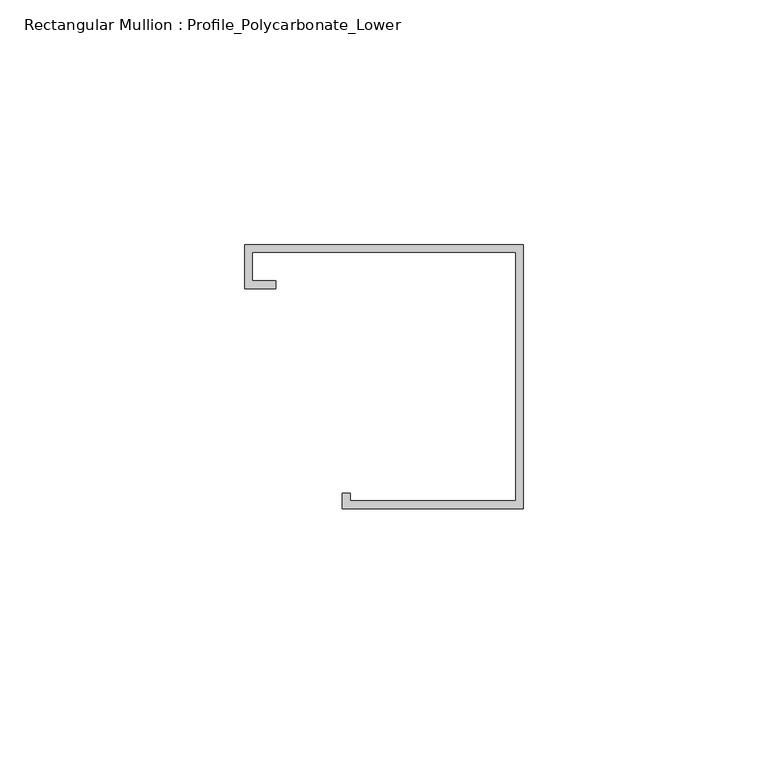
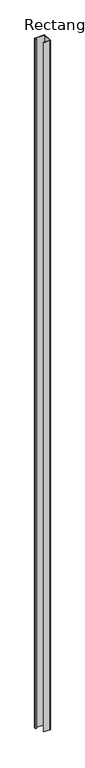
"""IFC4 building model written with IfcOpenShell, lengths in millimetres: member geometry, Rectangular Mullion : Profile_Polycarbonate_Lower."""

import ifcopenshell
import ifcopenshell.guid

model = None  # the IFC model being written
_history = None  # IfcOwnerHistory: only IFC2X3 demands one
_inside = {}  # id of a spatial element -> (the spatial element, [elements in it])
_under = {}  # id of a project, library or spatial element -> (it, [spatial elements below it])
_declared = {}  # id of a project -> (the project, [libraries it declares])
_typed = {}  # id of a type object -> (the type object, [elements of that type])
_made_of = {}  # id of a material, layer set ... -> (it, [elements and type objects made of it])


def new_model(schema):
    """Start an empty IFC model of exactly this schema.

    Asked for "IFC4X3", IfcOpenShell would pick the latest addendum, in which some entities
    have other attributes; the version numbers below select the first issue.
    IFC2X3 requires an IfcOwnerHistory on every rooted entity: one is made here for all.
    """
    global model, _history
    if schema == "IFC4X3":
        model = ifcopenshell.file(schema_version=(4, 3, 0, 0))
    else:
        model = ifcopenshell.file(schema=schema)
    _inside.clear()
    _under.clear()
    _declared.clear()
    _typed.clear()
    _made_of.clear()
    _history = None
    if model.schema == "IFC2X3":
        org = make("IfcOrganization", Name="unknown")
        user = make(
            "IfcPersonAndOrganization",
            ThePerson=make("IfcPerson", FamilyName="unknown"),
            TheOrganization=org,
        )
        app = make(
            "IfcApplication",
            ApplicationDeveloper=org,
            Version="unknown",
            ApplicationFullName="unknown",
            ApplicationIdentifier="unknown",
        )
        _history = make(
            "IfcOwnerHistory",
            OwningUser=user,
            OwningApplication=app,
            ChangeAction="ADDED",
            CreationDate=0,
        )
    return model


def make(cls, **values):
    """One entity of the class cls with the attributes given. An attribute that is None is left unset."""
    return model.create_entity(
        cls, **{name: value for name, value in values.items() if value is not None}
    )


def rooted(cls, **values):
    """An entity with a GlobalId (a new one), such as an element, a storey or a relation."""
    return make(cls, GlobalId=ifcopenshell.guid.new(), OwnerHistory=_history, **values)


def si_unit(unit_type, name, prefix=None):
    """IfcSIUnit, for example si_unit("LENGTHUNIT", "METRE", prefix="MILLI")."""
    return make("IfcSIUnit", UnitType=unit_type, Prefix=prefix, Name=name)


def assignment(units):
    """IfcUnitAssignment: the units of a project."""
    return None if units is None else make("IfcUnitAssignment", Units=units)


def point(xyz):
    """IfcCartesianPoint."""
    return None if xyz is None else make("IfcCartesianPoint", Coordinates=xyz)


def direction(xyz):
    """IfcDirection."""
    return None if xyz is None else make("IfcDirection", DirectionRatios=xyz)


def frame(location, z_axis=None, x_axis=None):
    """IfcAxis2Placement3D, a coordinate frame: its origin and axes. An axis left out is left unset."""
    return make(
        "IfcAxis2Placement3D",
        Location=point(location),
        Axis=direction(z_axis),
        RefDirection=direction(x_axis),
    )


def origin():
    """The frame at (0, 0, 0) with its axes left unset."""
    return frame((0.0, 0.0, 0.0))


def place(relative_to, where):
    """IfcLocalPlacement: puts the frame where relative to a parent placement (None: the world)."""
    return make(
        "IfcLocalPlacement", PlacementRelTo=relative_to, RelativePlacement=where
    )


def context(
    kind, dimensions, precision=None, world=None, true_north=None, identifier=None
):
    """IfcGeometricRepresentationContext, for example the 3D "Model" context."""
    return make(
        "IfcGeometricRepresentationContext",
        ContextIdentifier=identifier,
        ContextType=kind,
        CoordinateSpaceDimension=dimensions,
        Precision=precision,
        WorldCoordinateSystem=world,
        TrueNorth=true_north,
    )


def project(units=None, contexts=None):
    """IfcProject with its units and contexts."""
    return rooted(
        "IfcProject",
        Name="project",
        RepresentationContexts=contexts,
        UnitsInContext=assignment(units),
    )


def spatial(cls, under=None, at=None, **own):
    """A site, building, storey or space (cls), placed at a placement, below another one or the project."""
    s = rooted(cls, ObjectPlacement=at, **own)
    if under is not None:
        _under.setdefault(under.id(), (under, []))[1].append(s)
    return s


def polyline(points):
    """IfcPolyline through the points."""
    return make("IfcPolyline", Points=[point(p) for p in points])


def outline(outer, holes=None, kind="AREA"):
    """IfcArbitraryClosedProfileDef: a profile drawn as a closed curve; with holes, ...WithVoids."""
    if holes is None:
        return make("IfcArbitraryClosedProfileDef", ProfileType=kind, OuterCurve=outer)
    return make(
        "IfcArbitraryProfileDefWithVoids",
        ProfileType=kind,
        OuterCurve=outer,
        InnerCurves=holes,
    )


def extrude(swept, where, along, depth):
    """IfcExtrudedAreaSolid: the profile swept, set in the frame where, extruded along a direction by depth."""
    return make(
        "IfcExtrudedAreaSolid",
        SweptArea=swept,
        Position=where,
        ExtrudedDirection=direction(along),
        Depth=depth,
    )


def shape(context_of_items, identifier, shape_type, items):
    """IfcShapeRepresentation: the items that make up one representation, for example the "Body"."""
    return make(
        "IfcShapeRepresentation",
        ContextOfItems=context_of_items,
        RepresentationIdentifier=identifier,
        RepresentationType=shape_type,
        Items=items,
    )


def source(mapping_origin, context_of_items, identifier, shape_type, items):
    """IfcRepresentationMap: a shape defined once, which mapped items show again and again."""
    return make(
        "IfcRepresentationMap",
        MappingOrigin=mapping_origin,
        MappedRepresentation=shape(context_of_items, identifier, shape_type, items),
    )


def transform(
    local_origin,
    x_axis=None,
    y_axis=None,
    z_axis=None,
    scale=None,
    scale2=None,
    scale3=None,
    uniform=True,
):
    """IfcCartesianTransformationOperator3D, or its non-uniform kind. x_axis, y_axis, z_axis: its Axis1, 2, 3."""
    if uniform:
        return make(
            "IfcCartesianTransformationOperator3D",
            Axis1=direction(x_axis),
            Axis2=direction(y_axis),
            LocalOrigin=point(local_origin),
            Scale=scale,
            Axis3=direction(z_axis),
        )
    return make(
        "IfcCartesianTransformationOperator3DnonUniform",
        Axis1=direction(x_axis),
        Axis2=direction(y_axis),
        LocalOrigin=point(local_origin),
        Scale=scale,
        Axis3=direction(z_axis),
        Scale2=scale2,
        Scale3=scale3,
    )


def mapped(mapping_source, mapping_target):
    """IfcMappedItem: shows the shape of a source again, moved by a transform."""
    return make(
        "IfcMappedItem", MappingSource=mapping_source, MappingTarget=mapping_target
    )


def made_of(thing, what):
    """Note that an element or type object is made of a material, layer set ...; save() writes the relation."""
    if what is not None:
        _made_of.setdefault(what.id(), (what, []))[1].append(thing)
    return thing


def element(
    cls,
    number,
    at=None,
    inside=None,
    cuts=None,
    type_object=None,
    material=None,
    context=None,
    identifier="Body",
    shape_type=None,
    held_by="IfcProductDefinitionShape",
    body=None,
    shapes=None,
    **own,
):
    """One element of the class cls, such as IfcWall. Its Tag is "e" and its number.

    at: its placement. inside: the storey or other place that contains it. cuts: it is an
    opening in that element (IfcRelVoidsElement). A single representation is given by context,
    identifier, shape_type and body (its items); several are given by shapes. held_by: the class
    of the entity that holds the representations. save() writes the other relations.
    """
    e = rooted(cls, Tag="e%d" % number, ObjectPlacement=at, **own)
    if body is not None:
        shapes = [shape(context, identifier, shape_type, body)]
    if shapes is not None:
        e.Representation = make(held_by, Representations=shapes)
    if inside is not None:
        _inside.setdefault(inside.id(), (inside, []))[1].append(e)
    if cuts is not None:
        rooted(
            "IfcRelVoidsElement", RelatingBuildingElement=cuts, RelatedOpeningElement=e
        )
    if type_object is not None:
        _typed.setdefault(type_object.id(), (type_object, []))[1].append(e)
    return made_of(e, material)


def aggregate(whole, parts):
    """IfcRelAggregates: a whole, such as a stair, and the parts it consists of."""
    return rooted("IfcRelAggregates", RelatingObject=whole, RelatedObjects=parts)


def save(model, path):
    """Write the relations noted so far, then the file.

    IfcRelAggregates (storeys below a building ...), IfcRelContainedInSpatialStructure (elements
    in a storey), IfcRelDefinesByType, IfcRelAssociatesMaterial and IfcRelDeclares: one each for
    every whole, place, type object, material and project.
    """
    for whole, parts in _under.values():
        aggregate(whole, parts)
    for where, things in _inside.values():
        rooted(
            "IfcRelContainedInSpatialStructure",
            RelatedElements=things,
            RelatingStructure=where,
        )
    for kind, things in _typed.values():
        rooted("IfcRelDefinesByType", RelatedObjects=things, RelatingType=kind)
    for what, things in _made_of.values():
        rooted("IfcRelAssociatesMaterial", RelatedObjects=things, RelatingMaterial=what)
    for by, libraries in _declared.values():
        rooted("IfcRelDeclares", RelatingContext=by, RelatedDefinitions=libraries)
    model.write(path)


def rectangular_mullion_profile_polycarbonate_lower_07ae4ce1(model_context):
    return source(origin(), model_context, "Body", "SweptSolid", [
        extrude(outline(polyline([(0.0, 28.984575), (0.0, -25.015825), (-36.9824, -25.015825), (-36.9824, -21.840825), (-35.3949, -21.840825), (-35.3949, -23.428325), (-1.5875, -23.428325), (-1.5875, 27.397075), (-55.4101, 27.397075), (-55.4101, 21.580475), (-50.6476, 21.580475), (-50.6476, 19.992975), (-56.9976, 19.992975), (-56.9976, 28.984575), (0.0, 28.984575)])), frame((0.0, 0.0, -4116.6609733), z_axis=(0.0, 0.0, 1.0), x_axis=(1.0, 0.0, 0.0)), (0.0, 0.0, 1.0), 4116.6609733),
    ])


if __name__ == "__main__":
    model = new_model("IFC4")
    model_context = context("Model", 3, world=origin())
    ifc_project = project(units=[si_unit("LENGTHUNIT", "METRE", prefix="MILLI")], contexts=[model_context])
    site = spatial("IfcSite", under=ifc_project)
    building = spatial("IfcBuilding", under=site)
    placement = place(None, origin())
    rectangular_mullion_profile_polycarbonate_lower_shape = rectangular_mullion_profile_polycarbonate_lower_07ae4ce1(model_context)
    element("IfcMember", 1, ObjectType="Rectangular Mullion : Profile_Polycarbonate_Lower", at=placement, inside=building, context=model_context, shape_type="MappedRepresentation", body=[
        mapped(rectangular_mullion_profile_polycarbonate_lower_shape, transform((0.0, 0.0, 0.0), x_axis=(1.0, 0.0, 0.0), y_axis=(0.0, 1.0, 0.0), z_axis=(0.0, 0.0, 1.0))),
    ])
    save(model, "model.ifc")

# Revit data of these elements
# Type "Rectangular Mullion : Profile_Polycarbonate_Lower"
#   built-in parameter 1007322 = 0.177167 (stored number, unit not read)
#   built-in parameter 1007321 = 0 (stored number, unit not read)
#   built-in parameter 1007320 = 0.00520833 (stored number, unit not read)
